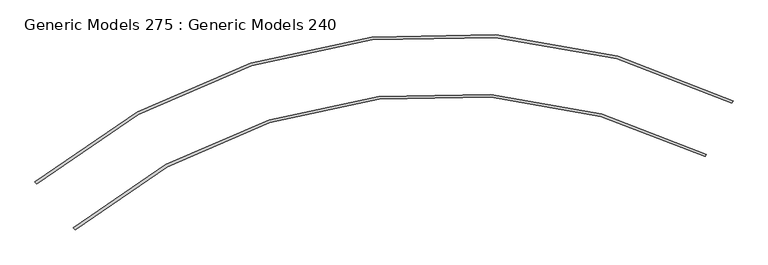
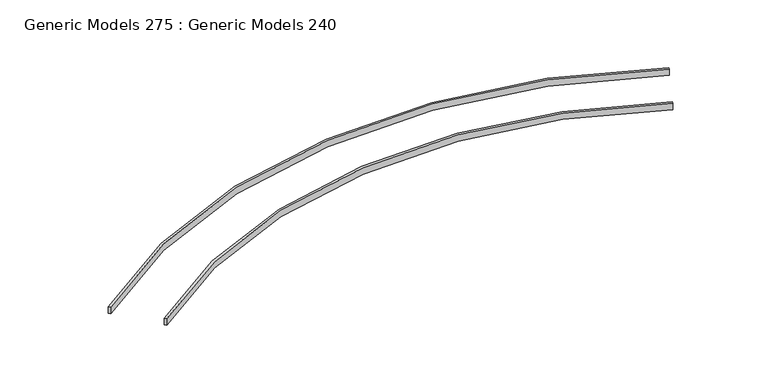
"""IFC4 building model written with IfcOpenShell, lengths in millimetres: proxy geometry, Generic Models 275 : Generic Models 240."""

import ifcopenshell
import ifcopenshell.guid

model = None  # the IFC model being written
_history = None  # IfcOwnerHistory: only IFC2X3 demands one
_inside = {}  # id of a spatial element -> (the spatial element, [elements in it])
_under = {}  # id of a project, library or spatial element -> (it, [spatial elements below it])
_declared = {}  # id of a project -> (the project, [libraries it declares])
_typed = {}  # id of a type object -> (the type object, [elements of that type])
_made_of = {}  # id of a material, layer set ... -> (it, [elements and type objects made of it])


def new_model(schema):
    """Start an empty IFC model of exactly this schema.

    Asked for "IFC4X3", IfcOpenShell would pick the latest addendum, in which some entities
    have other attributes; the version numbers below select the first issue.
    IFC2X3 requires an IfcOwnerHistory on every rooted entity: one is made here for all.
    """
    global model, _history
    if schema == "IFC4X3":
        model = ifcopenshell.file(schema_version=(4, 3, 0, 0))
    else:
        model = ifcopenshell.file(schema=schema)
    _inside.clear()
    _under.clear()
    _declared.clear()
    _typed.clear()
    _made_of.clear()
    _history = None
    if model.schema == "IFC2X3":
        org = make("IfcOrganization", Name="unknown")
        user = make(
            "IfcPersonAndOrganization",
            ThePerson=make("IfcPerson", FamilyName="unknown"),
            TheOrganization=org,
        )
        app = make(
            "IfcApplication",
            ApplicationDeveloper=org,
            Version="unknown",
            ApplicationFullName="unknown",
            ApplicationIdentifier="unknown",
        )
        _history = make(
            "IfcOwnerHistory",
            OwningUser=user,
            OwningApplication=app,
            ChangeAction="ADDED",
            CreationDate=0,
        )
    return model


def make(cls, **values):
    """One entity of the class cls with the attributes given. An attribute that is None is left unset."""
    return model.create_entity(
        cls, **{name: value for name, value in values.items() if value is not None}
    )


def rooted(cls, **values):
    """An entity with a GlobalId (a new one), such as an element, a storey or a relation."""
    return make(cls, GlobalId=ifcopenshell.guid.new(), OwnerHistory=_history, **values)


def si_unit(unit_type, name, prefix=None):
    """IfcSIUnit, for example si_unit("LENGTHUNIT", "METRE", prefix="MILLI")."""
    return make("IfcSIUnit", UnitType=unit_type, Prefix=prefix, Name=name)


def assignment(units):
    """IfcUnitAssignment: the units of a project."""
    return None if units is None else make("IfcUnitAssignment", Units=units)


def point(xyz):
    """IfcCartesianPoint."""
    return None if xyz is None else make("IfcCartesianPoint", Coordinates=xyz)


def direction(xyz):
    """IfcDirection."""
    return None if xyz is None else make("IfcDirection", DirectionRatios=xyz)


def frame(location, z_axis=None, x_axis=None):
    """IfcAxis2Placement3D, a coordinate frame: its origin and axes. An axis left out is left unset."""
    return make(
        "IfcAxis2Placement3D",
        Location=point(location),
        Axis=direction(z_axis),
        RefDirection=direction(x_axis),
    )


def frame_2d(location, x_axis=None):
    """IfcAxis2Placement2D, a coordinate frame in the plane: its origin and x axis."""
    return make(
        "IfcAxis2Placement2D", Location=point(location), RefDirection=direction(x_axis)
    )


def origin():
    """The frame at (0, 0, 0) with its axes left unset."""
    return frame((0.0, 0.0, 0.0))


def place(relative_to, where):
    """IfcLocalPlacement: puts the frame where relative to a parent placement (None: the world)."""
    return make(
        "IfcLocalPlacement", PlacementRelTo=relative_to, RelativePlacement=where
    )


def context(
    kind, dimensions, precision=None, world=None, true_north=None, identifier=None
):
    """IfcGeometricRepresentationContext, for example the 3D "Model" context."""
    return make(
        "IfcGeometricRepresentationContext",
        ContextIdentifier=identifier,
        ContextType=kind,
        CoordinateSpaceDimension=dimensions,
        Precision=precision,
        WorldCoordinateSystem=world,
        TrueNorth=true_north,
    )


def project(units=None, contexts=None):
    """IfcProject with its units and contexts."""
    return rooted(
        "IfcProject",
        Name="project",
        RepresentationContexts=contexts,
        UnitsInContext=assignment(units),
    )


def spatial(cls, under=None, at=None, **own):
    """A site, building, storey or space (cls), placed at a placement, below another one or the project."""
    s = rooted(cls, ObjectPlacement=at, **own)
    if under is not None:
        _under.setdefault(under.id(), (under, []))[1].append(s)
    return s


def polyline(points):
    """IfcPolyline through the points."""
    return make("IfcPolyline", Points=[point(p) for p in points])


def circle_curve(where, radius):
    """IfcCircle in the frame where."""
    return make("IfcCircle", Position=where, Radius=radius)


def trimmed(basis, trim1, trim2, sense, master):
    """IfcTrimmedCurve: the piece of a basis curve between two trims."""
    return make(
        "IfcTrimmedCurve",
        BasisCurve=basis,
        Trim1=trim1,
        Trim2=trim2,
        SenseAgreement=sense,
        MasterRepresentation=master,
    )


def segment(curve, same_sense, transition):
    """IfcCompositeCurveSegment."""
    return make(
        "IfcCompositeCurveSegment",
        Transition=transition,
        SameSense=same_sense,
        ParentCurve=curve,
    )


def composite_curve(segments, self_intersect=None):
    """IfcCompositeCurve: segments joined end to end."""
    return make("IfcCompositeCurve", Segments=segments, SelfIntersect=self_intersect)


def outline(outer, holes=None, kind="AREA"):
    """IfcArbitraryClosedProfileDef: a profile drawn as a closed curve; with holes, ...WithVoids."""
    if holes is None:
        return make("IfcArbitraryClosedProfileDef", ProfileType=kind, OuterCurve=outer)
    return make(
        "IfcArbitraryProfileDefWithVoids",
        ProfileType=kind,
        OuterCurve=outer,
        InnerCurves=holes,
    )


def extrude(swept, where, along, depth):
    """IfcExtrudedAreaSolid: the profile swept, set in the frame where, extruded along a direction by depth."""
    return make(
        "IfcExtrudedAreaSolid",
        SweptArea=swept,
        Position=where,
        ExtrudedDirection=direction(along),
        Depth=depth,
    )


def shape(context_of_items, identifier, shape_type, items):
    """IfcShapeRepresentation: the items that make up one representation, for example the "Body"."""
    return make(
        "IfcShapeRepresentation",
        ContextOfItems=context_of_items,
        RepresentationIdentifier=identifier,
        RepresentationType=shape_type,
        Items=items,
    )


def source(mapping_origin, context_of_items, identifier, shape_type, items):
    """IfcRepresentationMap: a shape defined once, which mapped items show again and again."""
    return make(
        "IfcRepresentationMap",
        MappingOrigin=mapping_origin,
        MappedRepresentation=shape(context_of_items, identifier, shape_type, items),
    )


def transform(
    local_origin,
    x_axis=None,
    y_axis=None,
    z_axis=None,
    scale=None,
    scale2=None,
    scale3=None,
    uniform=True,
):
    """IfcCartesianTransformationOperator3D, or its non-uniform kind. x_axis, y_axis, z_axis: its Axis1, 2, 3."""
    if uniform:
        return make(
            "IfcCartesianTransformationOperator3D",
            Axis1=direction(x_axis),
            Axis2=direction(y_axis),
            LocalOrigin=point(local_origin),
            Scale=scale,
            Axis3=direction(z_axis),
        )
    return make(
        "IfcCartesianTransformationOperator3DnonUniform",
        Axis1=direction(x_axis),
        Axis2=direction(y_axis),
        LocalOrigin=point(local_origin),
        Scale=scale,
        Axis3=direction(z_axis),
        Scale2=scale2,
        Scale3=scale3,
    )


def mapped(mapping_source, mapping_target):
    """IfcMappedItem: shows the shape of a source again, moved by a transform."""
    return make(
        "IfcMappedItem", MappingSource=mapping_source, MappingTarget=mapping_target
    )


def made_of(thing, what):
    """Note that an element or type object is made of a material, layer set ...; save() writes the relation."""
    if what is not None:
        _made_of.setdefault(what.id(), (what, []))[1].append(thing)
    return thing


def element(
    cls,
    number,
    at=None,
    inside=None,
    cuts=None,
    type_object=None,
    material=None,
    context=None,
    identifier="Body",
    shape_type=None,
    held_by="IfcProductDefinitionShape",
    body=None,
    shapes=None,
    **own,
):
    """One element of the class cls, such as IfcWall. Its Tag is "e" and its number.

    at: its placement. inside: the storey or other place that contains it. cuts: it is an
    opening in that element (IfcRelVoidsElement). A single representation is given by context,
    identifier, shape_type and body (its items); several are given by shapes. held_by: the class
    of the entity that holds the representations. save() writes the other relations.
    """
    e = rooted(cls, Tag="e%d" % number, ObjectPlacement=at, **own)
    if body is not None:
        shapes = [shape(context, identifier, shape_type, body)]
    if shapes is not None:
        e.Representation = make(held_by, Representations=shapes)
    if inside is not None:
        _inside.setdefault(inside.id(), (inside, []))[1].append(e)
    if cuts is not None:
        rooted(
            "IfcRelVoidsElement", RelatingBuildingElement=cuts, RelatedOpeningElement=e
        )
    if type_object is not None:
        _typed.setdefault(type_object.id(), (type_object, []))[1].append(e)
    return made_of(e, material)


def aggregate(whole, parts):
    """IfcRelAggregates: a whole, such as a stair, and the parts it consists of."""
    return rooted("IfcRelAggregates", RelatingObject=whole, RelatedObjects=parts)


def save(model, path):
    """Write the relations noted so far, then the file.

    IfcRelAggregates (storeys below a building ...), IfcRelContainedInSpatialStructure (elements
    in a storey), IfcRelDefinesByType, IfcRelAssociatesMaterial and IfcRelDeclares: one each for
    every whole, place, type object, material and project.
    """
    for whole, parts in _under.values():
        aggregate(whole, parts)
    for where, things in _inside.values():
        rooted(
            "IfcRelContainedInSpatialStructure",
            RelatedElements=things,
            RelatingStructure=where,
        )
    for kind, things in _typed.values():
        rooted("IfcRelDefinesByType", RelatedObjects=things, RelatingType=kind)
    for what, things in _made_of.values():
        rooted("IfcRelAssociatesMaterial", RelatedObjects=things, RelatingMaterial=what)
    for by, libraries in _declared.values():
        rooted("IfcRelDeclares", RelatingContext=by, RelatedDefinitions=libraries)
    model.write(path)


def generic_models_275_generic_models_240_07ee5088(model_context):
    return source(origin(), model_context, "Body", "SweptSolid", [
        extrude(outline(composite_curve([segment(trimmed(circle_curve(frame_2d((-832.04683, -25139.2753781)), 3119.9218919), [point((-2834.5318691, -22746.7941808))], [point((568.4611508, -22351.3567984))], False, "CARTESIAN"), True, "CONTINUOUS"), segment(polyline([(568.4611508, -22351.3567984), (562.7602224, -22362.7053408)]), True, "CONTINUOUS"), segment(trimmed(circle_curve(frame_2d((-832.04683, -25139.2753781)), 3107.2218919), [point((562.7602224, -22362.7053408))], [point((-2826.380524, -22756.53305))], True, "CARTESIAN"), True, "CONTINUOUS"), segment(polyline([(-2826.380524, -22756.53305), (-2834.5318691, -22746.7941808)]), True, "CONTINUOUS")], self_intersect=False)), frame((0.0, 0.0, 1035.05), z_axis=(0.0, 0.0, 1.0), x_axis=(1.0, 0.0, 0.0)), (0.0, 0.0, 1.0), 38.1),
        extrude(outline(composite_curve([segment(trimmed(circle_curve(frame_2d((-832.04683, -25139.2753781)), 2827.8218919), [point((-2647.050932, -22970.7881723))], [point((437.3397973, -22612.3732742))], False, "CARTESIAN"), True, "CONTINUOUS"), segment(polyline([(437.3397973, -22612.3732742), (431.6388689, -22623.7218166)]), True, "CONTINUOUS"), segment(trimmed(circle_curve(frame_2d((-832.04683, -25139.2753781)), 2815.1218919), [point((431.6388689, -22623.7218166))], [point((-2638.8995869, -22980.5270415))], True, "CARTESIAN"), True, "CONTINUOUS"), segment(polyline([(-2638.8995869, -22980.5270415), (-2647.050932, -22970.7881723)]), True, "CONTINUOUS")], self_intersect=False)), frame((0.0, 0.0, 1035.05), z_axis=(0.0, 0.0, 1.0), x_axis=(1.0, 0.0, 0.0)), (0.0, 0.0, 1.0), 38.1),
    ])


if __name__ == "__main__":
    model = new_model("IFC4")
    model_context = context("Model", 3, world=origin())
    ifc_project = project(units=[si_unit("LENGTHUNIT", "METRE", prefix="MILLI")], contexts=[model_context])
    site = spatial("IfcSite", under=ifc_project)
    building = spatial("IfcBuilding", under=site)
    placement = place(None, origin())
    generic_models_275_generic_models_240_shape = generic_models_275_generic_models_240_07ee5088(model_context)
    element("IfcBuildingElementProxy", 1, Name="Generic Models 275 : Generic Models 240", ObjectType="Generic Models 275 : Generic Models 240", at=placement, inside=building, context=model_context, shape_type="MappedRepresentation", body=[
        mapped(generic_models_275_generic_models_240_shape, transform((0.0, 0.0, 0.0), x_axis=(1.0, 0.0, 0.0), y_axis=(0.0, 1.0, 0.0), z_axis=(0.0, 0.0, 1.0))),
    ])
    save(model, "model.ifc")

# Revit data of these elements
# Element 1 (IfcBuildingElementProxy, "Generic Models 275 : Generic Models 240")
#   Materials on its faces: "1/2\" x 2\" TRIM BOARD"
# Materials
#   "1/2\" x 2\" TRIM BOARD": class "Wood", colour RGB 48 37 22, transparency 0, Description = "Pinus Echinata", Cost = 0
